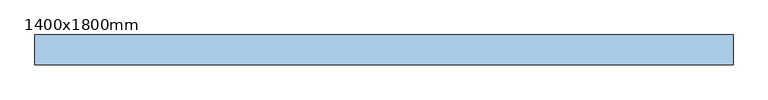
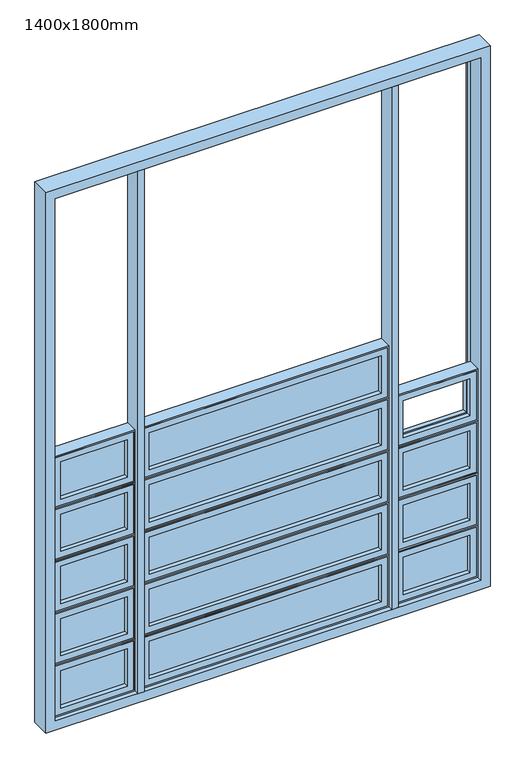
"""IFC4 building model written with IfcOpenShell, lengths in millimetres: window geometry, Janela Basculante 01 : 1400x1800mm."""

import ifcopenshell
import ifcopenshell.guid

model = None  # the IFC model being written
_history = None  # IfcOwnerHistory: only IFC2X3 demands one
_inside = {}  # id of a spatial element -> (the spatial element, [elements in it])
_under = {}  # id of a project, library or spatial element -> (it, [spatial elements below it])
_declared = {}  # id of a project -> (the project, [libraries it declares])
_typed = {}  # id of a type object -> (the type object, [elements of that type])
_made_of = {}  # id of a material, layer set ... -> (it, [elements and type objects made of it])


def new_model(schema):
    """Start an empty IFC model of exactly this schema.

    Asked for "IFC4X3", IfcOpenShell would pick the latest addendum, in which some entities
    have other attributes; the version numbers below select the first issue.
    IFC2X3 requires an IfcOwnerHistory on every rooted entity: one is made here for all.
    """
    global model, _history
    if schema == "IFC4X3":
        model = ifcopenshell.file(schema_version=(4, 3, 0, 0))
    else:
        model = ifcopenshell.file(schema=schema)
    _inside.clear()
    _under.clear()
    _declared.clear()
    _typed.clear()
    _made_of.clear()
    _history = None
    if model.schema == "IFC2X3":
        org = make("IfcOrganization", Name="unknown")
        user = make(
            "IfcPersonAndOrganization",
            ThePerson=make("IfcPerson", FamilyName="unknown"),
            TheOrganization=org,
        )
        app = make(
            "IfcApplication",
            ApplicationDeveloper=org,
            Version="unknown",
            ApplicationFullName="unknown",
            ApplicationIdentifier="unknown",
        )
        _history = make(
            "IfcOwnerHistory",
            OwningUser=user,
            OwningApplication=app,
            ChangeAction="ADDED",
            CreationDate=0,
        )
    return model


def make(cls, **values):
    """One entity of the class cls with the attributes given. An attribute that is None is left unset."""
    return model.create_entity(
        cls, **{name: value for name, value in values.items() if value is not None}
    )


def rooted(cls, **values):
    """An entity with a GlobalId (a new one), such as an element, a storey or a relation."""
    return make(cls, GlobalId=ifcopenshell.guid.new(), OwnerHistory=_history, **values)


def si_unit(unit_type, name, prefix=None):
    """IfcSIUnit, for example si_unit("LENGTHUNIT", "METRE", prefix="MILLI")."""
    return make("IfcSIUnit", UnitType=unit_type, Prefix=prefix, Name=name)


def assignment(units):
    """IfcUnitAssignment: the units of a project."""
    return None if units is None else make("IfcUnitAssignment", Units=units)


def point(xyz):
    """IfcCartesianPoint."""
    return None if xyz is None else make("IfcCartesianPoint", Coordinates=xyz)


def direction(xyz):
    """IfcDirection."""
    return None if xyz is None else make("IfcDirection", DirectionRatios=xyz)


def frame(location, z_axis=None, x_axis=None):
    """IfcAxis2Placement3D, a coordinate frame: its origin and axes. An axis left out is left unset."""
    return make(
        "IfcAxis2Placement3D",
        Location=point(location),
        Axis=direction(z_axis),
        RefDirection=direction(x_axis),
    )


def origin():
    """The frame at (0, 0, 0) with its axes left unset."""
    return frame((0.0, 0.0, 0.0))


def place(relative_to, where):
    """IfcLocalPlacement: puts the frame where relative to a parent placement (None: the world)."""
    return make(
        "IfcLocalPlacement", PlacementRelTo=relative_to, RelativePlacement=where
    )


def context(
    kind, dimensions, precision=None, world=None, true_north=None, identifier=None
):
    """IfcGeometricRepresentationContext, for example the 3D "Model" context."""
    return make(
        "IfcGeometricRepresentationContext",
        ContextIdentifier=identifier,
        ContextType=kind,
        CoordinateSpaceDimension=dimensions,
        Precision=precision,
        WorldCoordinateSystem=world,
        TrueNorth=true_north,
    )


def project(units=None, contexts=None):
    """IfcProject with its units and contexts."""
    return rooted(
        "IfcProject",
        Name="project",
        RepresentationContexts=contexts,
        UnitsInContext=assignment(units),
    )


def spatial(cls, under=None, at=None, **own):
    """A site, building, storey or space (cls), placed at a placement, below another one or the project."""
    s = rooted(cls, ObjectPlacement=at, **own)
    if under is not None:
        _under.setdefault(under.id(), (under, []))[1].append(s)
    return s


def polyline(points):
    """IfcPolyline through the points."""
    return make("IfcPolyline", Points=[point(p) for p in points])


def outline(outer, holes=None, kind="AREA"):
    """IfcArbitraryClosedProfileDef: a profile drawn as a closed curve; with holes, ...WithVoids."""
    if holes is None:
        return make("IfcArbitraryClosedProfileDef", ProfileType=kind, OuterCurve=outer)
    return make(
        "IfcArbitraryProfileDefWithVoids",
        ProfileType=kind,
        OuterCurve=outer,
        InnerCurves=holes,
    )


def extrude(swept, where, along, depth):
    """IfcExtrudedAreaSolid: the profile swept, set in the frame where, extruded along a direction by depth."""
    return make(
        "IfcExtrudedAreaSolid",
        SweptArea=swept,
        Position=where,
        ExtrudedDirection=direction(along),
        Depth=depth,
    )


def faces_of(points, faces, orient=None, outer=None):
    """IfcFace entities. A face is a list of loops; a loop is a list of indices into points, from 0.

    orient and outer hold one flag for each loop. By default every Orientation is true, the
    first loop of a face is its IfcFaceOuterBound and the others are IfcFaceBound.
    """
    made = []
    for i, loops in enumerate(faces):
        bounds = []
        for j, loop in enumerate(loops):
            is_outer = j == 0 if outer is None else outer[i][j]
            bounds.append(
                make(
                    "IfcFaceOuterBound" if is_outer else "IfcFaceBound",
                    Bound=make("IfcPolyLoop", Polygon=[points[k] for k in loop]),
                    Orientation=True if orient is None else orient[i][j],
                )
            )
        made.append(make("IfcFace", Bounds=bounds))
    return made


def faceted_brep(points, faces, orient=None, outer=None, voids=None):
    """IfcFacetedBrep: a solid bounded by flat faces; with voids (closed shells), ...WithVoids."""
    shared = [point(p) for p in points]
    hull = make("IfcClosedShell", CfsFaces=faces_of(shared, faces, orient, outer))
    if voids is None:
        return make("IfcFacetedBrep", Outer=hull)
    return make(
        "IfcFacetedBrepWithVoids",
        Outer=hull,
        Voids=[
            make(cls, CfsFaces=faces_of(shared, fs, o, b)) for cls, fs, o, b in voids
        ],
    )


def shape(context_of_items, identifier, shape_type, items):
    """IfcShapeRepresentation: the items that make up one representation, for example the "Body"."""
    return make(
        "IfcShapeRepresentation",
        ContextOfItems=context_of_items,
        RepresentationIdentifier=identifier,
        RepresentationType=shape_type,
        Items=items,
    )


def source(mapping_origin, context_of_items, identifier, shape_type, items):
    """IfcRepresentationMap: a shape defined once, which mapped items show again and again."""
    return make(
        "IfcRepresentationMap",
        MappingOrigin=mapping_origin,
        MappedRepresentation=shape(context_of_items, identifier, shape_type, items),
    )


def transform(
    local_origin,
    x_axis=None,
    y_axis=None,
    z_axis=None,
    scale=None,
    scale2=None,
    scale3=None,
    uniform=True,
):
    """IfcCartesianTransformationOperator3D, or its non-uniform kind. x_axis, y_axis, z_axis: its Axis1, 2, 3."""
    if uniform:
        return make(
            "IfcCartesianTransformationOperator3D",
            Axis1=direction(x_axis),
            Axis2=direction(y_axis),
            LocalOrigin=point(local_origin),
            Scale=scale,
            Axis3=direction(z_axis),
        )
    return make(
        "IfcCartesianTransformationOperator3DnonUniform",
        Axis1=direction(x_axis),
        Axis2=direction(y_axis),
        LocalOrigin=point(local_origin),
        Scale=scale,
        Axis3=direction(z_axis),
        Scale2=scale2,
        Scale3=scale3,
    )


def mapped(mapping_source, mapping_target):
    """IfcMappedItem: shows the shape of a source again, moved by a transform."""
    return make(
        "IfcMappedItem", MappingSource=mapping_source, MappingTarget=mapping_target
    )


def made_of(thing, what):
    """Note that an element or type object is made of a material, layer set ...; save() writes the relation."""
    if what is not None:
        _made_of.setdefault(what.id(), (what, []))[1].append(thing)
    return thing


def element(
    cls,
    number,
    at=None,
    inside=None,
    cuts=None,
    type_object=None,
    material=None,
    context=None,
    identifier="Body",
    shape_type=None,
    held_by="IfcProductDefinitionShape",
    body=None,
    shapes=None,
    **own,
):
    """One element of the class cls, such as IfcWall. Its Tag is "e" and its number.

    at: its placement. inside: the storey or other place that contains it. cuts: it is an
    opening in that element (IfcRelVoidsElement). A single representation is given by context,
    identifier, shape_type and body (its items); several are given by shapes. held_by: the class
    of the entity that holds the representations. save() writes the other relations.
    """
    e = rooted(cls, Tag="e%d" % number, ObjectPlacement=at, **own)
    if body is not None:
        shapes = [shape(context, identifier, shape_type, body)]
    if shapes is not None:
        e.Representation = make(held_by, Representations=shapes)
    if inside is not None:
        _inside.setdefault(inside.id(), (inside, []))[1].append(e)
    if cuts is not None:
        rooted(
            "IfcRelVoidsElement", RelatingBuildingElement=cuts, RelatedOpeningElement=e
        )
    if type_object is not None:
        _typed.setdefault(type_object.id(), (type_object, []))[1].append(e)
    return made_of(e, material)


def aggregate(whole, parts):
    """IfcRelAggregates: a whole, such as a stair, and the parts it consists of."""
    return rooted("IfcRelAggregates", RelatingObject=whole, RelatedObjects=parts)


def save(model, path):
    """Write the relations noted so far, then the file.

    IfcRelAggregates (storeys below a building ...), IfcRelContainedInSpatialStructure (elements
    in a storey), IfcRelDefinesByType, IfcRelAssociatesMaterial and IfcRelDeclares: one each for
    every whole, place, type object, material and project.
    """
    for whole, parts in _under.values():
        aggregate(whole, parts)
    for where, things in _inside.values():
        rooted(
            "IfcRelContainedInSpatialStructure",
            RelatedElements=things,
            RelatingStructure=where,
        )
    for kind, things in _typed.values():
        rooted("IfcRelDefinesByType", RelatedObjects=things, RelatingType=kind)
    for what, things in _made_of.values():
        rooted("IfcRelAssociatesMaterial", RelatedObjects=things, RelatingMaterial=what)
    for by, libraries in _declared.values():
        rooted("IfcRelDeclares", RelatingContext=by, RelatedDefinitions=libraries)
    model.write(path)


def window_1400x1800mm_1618d2dc(model_context):
    return source(origin(), model_context, "Body", "SolidModel", [
        faceted_brep([(435.0, -50.6, 1251.0), (435.0, -50.6, 1127.0), (435.0, -36.6, 1127.0), (435.0, -36.6, 1251.0), (428.0, -36.6, 1258.0), (428.0, -36.6, 1120.0), (428.0, -29.6, 1120.0), (428.0, -29.6, 1258.0), (435.0, -29.6, 1251.0), (435.0, -29.6, 1127.0), (435.0, -15.6, 1127.0), (435.0, -15.6, 1251.0), (415.0, -15.6, 1271.0), (415.0, -15.6, 1107.0), (415.0, -50.6, 1107.0), (415.0, -50.6, 1271.0), (645.0, -50.6, 1127.0), (645.0, -36.6, 1127.0), (652.0, -36.6, 1120.0), (652.0, -29.6, 1120.0), (645.0, -29.6, 1127.0), (645.0, -15.6, 1127.0), (665.0, -15.6, 1107.0), (665.0, -50.6, 1107.0), (645.0, -50.6, 1251.0), (645.0, -36.6, 1251.0), (652.0, -36.6, 1258.0), (652.0, -29.6, 1258.0), (645.0, -29.6, 1251.0), (645.0, -15.6, 1251.0), (665.0, -15.6, 1271.0), (665.0, -50.6, 1271.0)], [[[0, 1, 2, 3]], [[4, 5, 6, 7]], [[8, 9, 10, 11]], [[12, 13, 14, 15]], [[1, 16, 17, 2]], [[5, 18, 19, 6]], [[9, 20, 21, 10]], [[13, 22, 23, 14]], [[16, 24, 25, 17]], [[18, 26, 27, 19]], [[20, 28, 29, 21]], [[22, 30, 31, 23]], [[15, 14, 23, 31], [1, 0, 24, 16]], [[24, 0, 3, 25]], [[5, 4, 26, 18], [3, 2, 17, 25]], [[26, 4, 7, 27]], [[7, 6, 19, 27], [9, 8, 28, 20]], [[28, 8, 11, 29]], [[13, 12, 30, 22], [11, 10, 21, 29]], [[30, 12, 15, 31]]]),
        faceted_brep([(415.0, -50.6, 1271.0), (415.0, -50.6, 1107.0), (415.0, -15.6, 1107.0), (415.0, -15.6, 1271.0), (420.0, -15.6, 1266.0), (420.0, -15.6, 1112.0), (420.0, -10.6, 1112.0), (420.0, -10.6, 1266.0), (410.0, -10.6, 1276.0), (410.0, -10.6, 1102.0), (410.0, -50.6, 1102.0), (410.0, -50.6, 1276.0), (665.0, -50.6, 1107.0), (665.0, -15.6, 1107.0), (660.0, -15.6, 1112.0), (660.0, -10.6, 1112.0), (670.0, -10.6, 1102.0), (670.0, -50.6, 1102.0), (665.0, -50.6, 1271.0), (665.0, -15.6, 1271.0), (660.0, -15.6, 1266.0), (660.0, -10.6, 1266.0), (670.0, -10.6, 1276.0), (670.0, -50.6, 1276.0)], [[[0, 1, 2, 3]], [[4, 5, 6, 7]], [[8, 9, 10, 11]], [[1, 12, 13, 2]], [[5, 14, 15, 6]], [[9, 16, 17, 10]], [[12, 18, 19, 13]], [[14, 20, 21, 15]], [[16, 22, 23, 17]], [[11, 10, 17, 23], [1, 0, 18, 12]], [[18, 0, 3, 19]], [[3, 2, 13, 19], [5, 4, 20, 14]], [[20, 4, 7, 21]], [[9, 8, 22, 16], [7, 6, 15, 21]], [[22, 8, 11, 23]]]),
        extrude(outline(polyline([(652.0, -29.6), (652.0, -36.6), (428.0, -36.6), (428.0, -29.6), (652.0, -29.6)])), frame((0.0, 0.0, 946.0), z_axis=(0.0, 0.0, 1.0), x_axis=(1.0, 0.0, 0.0)), (0.0, 0.0, 1.0), 138.0),
        faceted_brep([(435.0, -50.6, 1077.0), (435.0, -50.6, 953.0), (435.0, -36.6, 953.0), (435.0, -36.6, 1077.0), (428.0, -36.6, 1084.0), (428.0, -36.6, 946.0), (428.0, -29.6, 946.0), (428.0, -29.6, 1084.0), (435.0, -29.6, 1077.0), (435.0, -29.6, 953.0), (435.0, -15.6, 953.0), (435.0, -15.6, 1077.0), (415.0, -15.6, 1097.0), (415.0, -15.6, 933.0), (415.0, -50.6, 933.0), (415.0, -50.6, 1097.0), (645.0, -50.6, 953.0), (645.0, -36.6, 953.0), (652.0, -36.6, 946.0), (652.0, -29.6, 946.0), (645.0, -29.6, 953.0), (645.0, -15.6, 953.0), (665.0, -15.6, 933.0), (665.0, -50.6, 933.0), (645.0, -50.6, 1077.0), (645.0, -36.6, 1077.0), (652.0, -36.6, 1084.0), (652.0, -29.6, 1084.0), (645.0, -29.6, 1077.0), (645.0, -15.6, 1077.0), (665.0, -15.6, 1097.0), (665.0, -50.6, 1097.0)], [[[0, 1, 2, 3]], [[4, 5, 6, 7]], [[8, 9, 10, 11]], [[12, 13, 14, 15]], [[1, 16, 17, 2]], [[5, 18, 19, 6]], [[9, 20, 21, 10]], [[13, 22, 23, 14]], [[16, 24, 25, 17]], [[18, 26, 27, 19]], [[20, 28, 29, 21]], [[22, 30, 31, 23]], [[15, 14, 23, 31], [1, 0, 24, 16]], [[24, 0, 3, 25]], [[5, 4, 26, 18], [3, 2, 17, 25]], [[26, 4, 7, 27]], [[7, 6, 19, 27], [9, 8, 28, 20]], [[28, 8, 11, 29]], [[13, 12, 30, 22], [11, 10, 21, 29]], [[30, 12, 15, 31]]]),
        faceted_brep([(415.0, -50.6, 1097.0), (415.0, -50.6, 933.0), (415.0, -15.6, 933.0), (415.0, -15.6, 1097.0), (420.0, -15.6, 1092.0), (420.0, -15.6, 938.0), (420.0, -10.6, 938.0), (420.0, -10.6, 1092.0), (410.0, -10.6, 1102.0), (410.0, -10.6, 928.0), (410.0, -50.6, 928.0), (410.0, -50.6, 1102.0), (665.0, -50.6, 933.0), (665.0, -15.6, 933.0), (660.0, -15.6, 938.0), (660.0, -10.6, 938.0), (670.0, -10.6, 928.0), (670.0, -50.6, 928.0), (665.0, -50.6, 1097.0), (665.0, -15.6, 1097.0), (660.0, -15.6, 1092.0), (660.0, -10.6, 1092.0), (670.0, -10.6, 1102.0), (670.0, -50.6, 1102.0)], [[[0, 1, 2, 3]], [[4, 5, 6, 7]], [[8, 9, 10, 11]], [[1, 12, 13, 2]], [[5, 14, 15, 6]], [[9, 16, 17, 10]], [[12, 18, 19, 13]], [[14, 20, 21, 15]], [[16, 22, 23, 17]], [[11, 10, 17, 23], [1, 0, 18, 12]], [[18, 0, 3, 19]], [[3, 2, 13, 19], [5, 4, 20, 14]], [[20, 4, 7, 21]], [[9, 8, 22, 16], [7, 6, 15, 21]], [[22, 8, 11, 23]]]),
        extrude(outline(polyline([(-372.0, -29.6), (372.0, -29.6), (372.0, -36.6), (-372.0, -36.6), (-372.0, -29.6)])), frame((0.0, 0.0, 1294.0), z_axis=(0.0, 0.0, 1.0), x_axis=(1.0, 0.0, 0.0)), (0.0, 0.0, 1.0), 138.0),
        faceted_brep([(365.0, -50.6, 1425.0), (365.0, -36.6, 1425.0), (365.0, -36.6, 1301.0), (365.0, -50.6, 1301.0), (372.0, -36.6, 1432.0), (372.0, -29.6, 1432.0), (372.0, -29.6, 1294.0), (372.0, -36.6, 1294.0), (365.0, -29.6, 1425.0), (365.0, -15.6, 1425.0), (365.0, -15.6, 1301.0), (365.0, -29.6, 1301.0), (385.0, -15.6, 1445.0), (385.0, -50.6, 1445.0), (385.0, -50.6, 1281.0), (385.0, -15.6, 1281.0), (-365.0, -36.6, 1301.0), (-365.0, -50.6, 1301.0), (-372.0, -29.6, 1294.0), (-372.0, -36.6, 1294.0), (-365.0, -15.6, 1301.0), (-365.0, -29.6, 1301.0), (-385.0, -50.6, 1281.0), (-385.0, -15.6, 1281.0), (-365.0, -36.6, 1425.0), (-365.0, -50.6, 1425.0), (-372.0, -29.6, 1432.0), (-372.0, -36.6, 1432.0), (-365.0, -15.6, 1425.0), (-365.0, -29.6, 1425.0), (-385.0, -50.6, 1445.0), (-385.0, -15.6, 1445.0)], [[[0, 1, 2, 3]], [[4, 5, 6, 7]], [[8, 9, 10, 11]], [[12, 13, 14, 15]], [[3, 2, 16, 17]], [[7, 6, 18, 19]], [[11, 10, 20, 21]], [[15, 14, 22, 23]], [[17, 16, 24, 25]], [[19, 18, 26, 27]], [[21, 20, 28, 29]], [[23, 22, 30, 31]], [[13, 30, 22, 14], [3, 17, 25, 0]], [[25, 24, 1, 0]], [[7, 19, 27, 4], [1, 24, 16, 2]], [[27, 26, 5, 4]], [[5, 26, 18, 6], [11, 21, 29, 8]], [[29, 28, 9, 8]], [[15, 23, 31, 12], [9, 28, 20, 10]], [[31, 30, 13, 12]]]),
        faceted_brep([(385.0, -50.6, 1445.0), (385.0, -15.6, 1445.0), (385.0, -15.6, 1281.0), (385.0, -50.6, 1281.0), (380.0, -15.6, 1440.0), (380.0, -10.6, 1440.0), (380.0, -10.6, 1286.0), (380.0, -15.6, 1286.0), (390.0, -10.6, 1450.0), (390.0, -50.6, 1450.0), (390.0, -50.6, 1276.0), (390.0, -10.6, 1276.0), (-385.0, -15.6, 1281.0), (-385.0, -50.6, 1281.0), (-380.0, -10.6, 1286.0), (-380.0, -15.6, 1286.0), (-390.0, -50.6, 1276.0), (-390.0, -10.6, 1276.0), (-385.0, -15.6, 1445.0), (-385.0, -50.6, 1445.0), (-380.0, -10.6, 1440.0), (-380.0, -15.6, 1440.0), (-390.0, -50.6, 1450.0), (-390.0, -10.6, 1450.0)], [[[0, 1, 2, 3]], [[4, 5, 6, 7]], [[8, 9, 10, 11]], [[3, 2, 12, 13]], [[7, 6, 14, 15]], [[11, 10, 16, 17]], [[13, 12, 18, 19]], [[15, 14, 20, 21]], [[17, 16, 22, 23]], [[9, 22, 16, 10], [3, 13, 19, 0]], [[19, 18, 1, 0]], [[1, 18, 12, 2], [7, 15, 21, 4]], [[21, 20, 5, 4]], [[11, 17, 23, 8], [5, 20, 14, 6]], [[23, 22, 9, 8]]]),
        extrude(outline(polyline([(-372.0, -29.6), (372.0, -29.6), (372.0, -36.6), (-372.0, -36.6), (-372.0, -29.6)])), frame((0.0, 0.0, 1120.0), z_axis=(0.0, 0.0, 1.0), x_axis=(1.0, 0.0, 0.0)), (0.0, 0.0, 1.0), 138.0),
        faceted_brep([(365.0, -50.6, 1251.0), (365.0, -36.6, 1251.0), (365.0, -36.6, 1127.0), (365.0, -50.6, 1127.0), (372.0, -36.6, 1258.0), (372.0, -29.6, 1258.0), (372.0, -29.6, 1120.0), (372.0, -36.6, 1120.0), (365.0, -29.6, 1251.0), (365.0, -15.6, 1251.0), (365.0, -15.6, 1127.0), (365.0, -29.6, 1127.0), (385.0, -15.6, 1271.0), (385.0, -50.6, 1271.0), (385.0, -50.6, 1107.0), (385.0, -15.6, 1107.0), (-365.0, -36.6, 1127.0), (-365.0, -50.6, 1127.0), (-372.0, -29.6, 1120.0), (-372.0, -36.6, 1120.0), (-365.0, -15.6, 1127.0), (-365.0, -29.6, 1127.0), (-385.0, -50.6, 1107.0), (-385.0, -15.6, 1107.0), (-365.0, -36.6, 1251.0), (-365.0, -50.6, 1251.0), (-372.0, -29.6, 1258.0), (-372.0, -36.6, 1258.0), (-365.0, -15.6, 1251.0), (-365.0, -29.6, 1251.0), (-385.0, -50.6, 1271.0), (-385.0, -15.6, 1271.0)], [[[0, 1, 2, 3]], [[4, 5, 6, 7]], [[8, 9, 10, 11]], [[12, 13, 14, 15]], [[3, 2, 16, 17]], [[7, 6, 18, 19]], [[11, 10, 20, 21]], [[15, 14, 22, 23]], [[17, 16, 24, 25]], [[19, 18, 26, 27]], [[21, 20, 28, 29]], [[23, 22, 30, 31]], [[13, 30, 22, 14], [3, 17, 25, 0]], [[25, 24, 1, 0]], [[7, 19, 27, 4], [1, 24, 16, 2]], [[27, 26, 5, 4]], [[5, 26, 18, 6], [11, 21, 29, 8]], [[29, 28, 9, 8]], [[15, 23, 31, 12], [9, 28, 20, 10]], [[31, 30, 13, 12]]]),
        faceted_brep([(385.0, -50.6, 1271.0), (385.0, -15.6, 1271.0), (385.0, -15.6, 1107.0), (385.0, -50.6, 1107.0), (380.0, -15.6, 1266.0), (380.0, -10.6, 1266.0), (380.0, -10.6, 1112.0), (380.0, -15.6, 1112.0), (390.0, -10.6, 1276.0), (390.0, -50.6, 1276.0), (390.0, -50.6, 1102.0), (390.0, -10.6, 1102.0), (-385.0, -15.6, 1107.0), (-385.0, -50.6, 1107.0), (-380.0, -10.6, 1112.0), (-380.0, -15.6, 1112.0), (-390.0, -50.6, 1102.0), (-390.0, -10.6, 1102.0), (-385.0, -15.6, 1271.0), (-385.0, -50.6, 1271.0), (-380.0, -10.6, 1266.0), (-380.0, -15.6, 1266.0), (-390.0, -50.6, 1276.0), (-390.0, -10.6, 1276.0)], [[[0, 1, 2, 3]], [[4, 5, 6, 7]], [[8, 9, 10, 11]], [[3, 2, 12, 13]], [[7, 6, 14, 15]], [[11, 10, 16, 17]], [[13, 12, 18, 19]], [[15, 14, 20, 21]], [[17, 16, 22, 23]], [[9, 22, 16, 10], [3, 13, 19, 0]], [[19, 18, 1, 0]], [[1, 18, 12, 2], [7, 15, 21, 4]], [[21, 20, 5, 4]], [[11, 17, 23, 8], [5, 20, 14, 6]], [[23, 22, 9, 8]]]),
        extrude(outline(polyline([(-372.0, -29.6), (372.0, -29.6), (372.0, -36.6), (-372.0, -36.6), (-372.0, -29.6)])), frame((0.0, 0.0, 946.0), z_axis=(0.0, 0.0, 1.0), x_axis=(1.0, 0.0, 0.0)), (0.0, 0.0, 1.0), 138.0),
        faceted_brep([(365.0, -50.6, 1077.0), (365.0, -36.6, 1077.0), (365.0, -36.6, 953.0), (365.0, -50.6, 953.0), (372.0, -36.6, 1084.0), (372.0, -29.6, 1084.0), (372.0, -29.6, 946.0), (372.0, -36.6, 946.0), (365.0, -29.6, 1077.0), (365.0, -15.6, 1077.0), (365.0, -15.6, 953.0), (365.0, -29.6, 953.0), (385.0, -15.6, 1097.0), (385.0, -50.6, 1097.0), (385.0, -50.6, 933.0), (385.0, -15.6, 933.0), (-365.0, -36.6, 953.0), (-365.0, -50.6, 953.0), (-372.0, -29.6, 946.0), (-372.0, -36.6, 946.0), (-365.0, -15.6, 953.0), (-365.0, -29.6, 953.0), (-385.0, -50.6, 933.0), (-385.0, -15.6, 933.0), (-365.0, -36.6, 1077.0), (-365.0, -50.6, 1077.0), (-372.0, -29.6, 1084.0), (-372.0, -36.6, 1084.0), (-365.0, -15.6, 1077.0), (-365.0, -29.6, 1077.0), (-385.0, -50.6, 1097.0), (-385.0, -15.6, 1097.0)], [[[0, 1, 2, 3]], [[4, 5, 6, 7]], [[8, 9, 10, 11]], [[12, 13, 14, 15]], [[3, 2, 16, 17]], [[7, 6, 18, 19]], [[11, 10, 20, 21]], [[15, 14, 22, 23]], [[17, 16, 24, 25]], [[19, 18, 26, 27]], [[21, 20, 28, 29]], [[23, 22, 30, 31]], [[13, 30, 22, 14], [3, 17, 25, 0]], [[25, 24, 1, 0]], [[7, 19, 27, 4], [1, 24, 16, 2]], [[27, 26, 5, 4]], [[5, 26, 18, 6], [11, 21, 29, 8]], [[29, 28, 9, 8]], [[15, 23, 31, 12], [9, 28, 20, 10]], [[31, 30, 13, 12]]]),
        faceted_brep([(385.0, -50.6, 1097.0), (385.0, -15.6, 1097.0), (385.0, -15.6, 933.0), (385.0, -50.6, 933.0), (380.0, -15.6, 1092.0), (380.0, -10.6, 1092.0), (380.0, -10.6, 938.0), (380.0, -15.6, 938.0), (390.0, -10.6, 1102.0), (390.0, -50.6, 1102.0), (390.0, -50.6, 928.0), (390.0, -10.6, 928.0), (-385.0, -15.6, 933.0), (-385.0, -50.6, 933.0), (-380.0, -10.6, 938.0), (-380.0, -15.6, 938.0), (-390.0, -50.6, 928.0), (-390.0, -10.6, 928.0), (-385.0, -15.6, 1097.0), (-385.0, -50.6, 1097.0), (-380.0, -10.6, 1092.0), (-380.0, -15.6, 1092.0), (-390.0, -50.6, 1102.0), (-390.0, -10.6, 1102.0)], [[[0, 1, 2, 3]], [[4, 5, 6, 7]], [[8, 9, 10, 11]], [[3, 2, 12, 13]], [[7, 6, 14, 15]], [[11, 10, 16, 17]], [[13, 12, 18, 19]], [[15, 14, 20, 21]], [[17, 16, 22, 23]], [[9, 22, 16, 10], [3, 13, 19, 0]], [[19, 18, 1, 0]], [[1, 18, 12, 2], [7, 15, 21, 4]], [[21, 20, 5, 4]], [[11, 17, 23, 8], [5, 20, 14, 6]], [[23, 22, 9, 8]]]),
        extrude(outline(polyline([(-428.0, -29.6), (-428.0, -36.6), (-652.0, -36.6), (-652.0, -29.6), (-428.0, -29.6)])), frame((0.0, 0.0, 1294.0), z_axis=(0.0, 0.0, 1.0), x_axis=(1.0, 0.0, 0.0)), (0.0, 0.0, 1.0), 138.0),
        faceted_brep([(-645.0, -50.6, 1425.0), (-645.0, -50.6, 1301.0), (-645.0, -36.6, 1301.0), (-645.0, -36.6, 1425.0), (-652.0, -36.6, 1432.0), (-652.0, -36.6, 1294.0), (-652.0, -29.6, 1294.0), (-652.0, -29.6, 1432.0), (-645.0, -29.6, 1425.0), (-645.0, -29.6, 1301.0), (-645.0, -15.6, 1301.0), (-645.0, -15.6, 1425.0), (-665.0, -15.6, 1445.0), (-665.0, -15.6, 1281.0), (-665.0, -50.6, 1281.0), (-665.0, -50.6, 1445.0), (-435.0, -50.6, 1301.0), (-435.0, -36.6, 1301.0), (-428.0, -36.6, 1294.0), (-428.0, -29.6, 1294.0), (-435.0, -29.6, 1301.0), (-435.0, -15.6, 1301.0), (-415.0, -15.6, 1281.0), (-415.0, -50.6, 1281.0), (-435.0, -50.6, 1425.0), (-435.0, -36.6, 1425.0), (-428.0, -36.6, 1432.0), (-428.0, -29.6, 1432.0), (-435.0, -29.6, 1425.0), (-435.0, -15.6, 1425.0), (-415.0, -15.6, 1445.0), (-415.0, -50.6, 1445.0)], [[[0, 1, 2, 3]], [[4, 5, 6, 7]], [[8, 9, 10, 11]], [[12, 13, 14, 15]], [[1, 16, 17, 2]], [[5, 18, 19, 6]], [[9, 20, 21, 10]], [[13, 22, 23, 14]], [[16, 24, 25, 17]], [[18, 26, 27, 19]], [[20, 28, 29, 21]], [[22, 30, 31, 23]], [[15, 14, 23, 31], [1, 0, 24, 16]], [[24, 0, 3, 25]], [[5, 4, 26, 18], [3, 2, 17, 25]], [[26, 4, 7, 27]], [[7, 6, 19, 27], [9, 8, 28, 20]], [[28, 8, 11, 29]], [[13, 12, 30, 22], [11, 10, 21, 29]], [[30, 12, 15, 31]]]),
        faceted_brep([(-665.0, -50.6, 1445.0), (-665.0, -50.6, 1281.0), (-665.0, -15.6, 1281.0), (-665.0, -15.6, 1445.0), (-660.0, -15.6, 1440.0), (-660.0, -15.6, 1286.0), (-660.0, -10.6, 1286.0), (-660.0, -10.6, 1440.0), (-670.0, -10.6, 1450.0), (-670.0, -10.6, 1276.0), (-670.0, -50.6, 1276.0), (-670.0, -50.6, 1450.0), (-415.0, -50.6, 1281.0), (-415.0, -15.6, 1281.0), (-420.0, -15.6, 1286.0), (-420.0, -10.6, 1286.0), (-410.0, -10.6, 1276.0), (-410.0, -50.6, 1276.0), (-415.0, -50.6, 1445.0), (-415.0, -15.6, 1445.0), (-420.0, -15.6, 1440.0), (-420.0, -10.6, 1440.0), (-410.0, -10.6, 1450.0), (-410.0, -50.6, 1450.0)], [[[0, 1, 2, 3]], [[4, 5, 6, 7]], [[8, 9, 10, 11]], [[1, 12, 13, 2]], [[5, 14, 15, 6]], [[9, 16, 17, 10]], [[12, 18, 19, 13]], [[14, 20, 21, 15]], [[16, 22, 23, 17]], [[11, 10, 17, 23], [1, 0, 18, 12]], [[18, 0, 3, 19]], [[3, 2, 13, 19], [5, 4, 20, 14]], [[20, 4, 7, 21]], [[9, 8, 22, 16], [7, 6, 15, 21]], [[22, 8, 11, 23]]]),
        extrude(outline(polyline([(-428.0, -29.6), (-428.0, -36.6), (-652.0, -36.6), (-652.0, -29.6), (-428.0, -29.6)])), frame((0.0, 0.0, 1120.0), z_axis=(0.0, 0.0, 1.0), x_axis=(1.0, 0.0, 0.0)), (0.0, 0.0, 1.0), 138.0),
        faceted_brep([(-645.0, -50.6, 1251.0), (-645.0, -50.6, 1127.0), (-645.0, -36.6, 1127.0), (-645.0, -36.6, 1251.0), (-652.0, -36.6, 1258.0), (-652.0, -36.6, 1120.0), (-652.0, -29.6, 1120.0), (-652.0, -29.6, 1258.0), (-645.0, -29.6, 1251.0), (-645.0, -29.6, 1127.0), (-645.0, -15.6, 1127.0), (-645.0, -15.6, 1251.0), (-665.0, -15.6, 1271.0), (-665.0, -15.6, 1107.0), (-665.0, -50.6, 1107.0), (-665.0, -50.6, 1271.0), (-435.0, -50.6, 1127.0), (-435.0, -36.6, 1127.0), (-428.0, -36.6, 1120.0), (-428.0, -29.6, 1120.0), (-435.0, -29.6, 1127.0), (-435.0, -15.6, 1127.0), (-415.0, -15.6, 1107.0), (-415.0, -50.6, 1107.0), (-435.0, -50.6, 1251.0), (-435.0, -36.6, 1251.0), (-428.0, -36.6, 1258.0), (-428.0, -29.6, 1258.0), (-435.0, -29.6, 1251.0), (-435.0, -15.6, 1251.0), (-415.0, -15.6, 1271.0), (-415.0, -50.6, 1271.0)], [[[0, 1, 2, 3]], [[4, 5, 6, 7]], [[8, 9, 10, 11]], [[12, 13, 14, 15]], [[1, 16, 17, 2]], [[5, 18, 19, 6]], [[9, 20, 21, 10]], [[13, 22, 23, 14]], [[16, 24, 25, 17]], [[18, 26, 27, 19]], [[20, 28, 29, 21]], [[22, 30, 31, 23]], [[15, 14, 23, 31], [1, 0, 24, 16]], [[24, 0, 3, 25]], [[5, 4, 26, 18], [3, 2, 17, 25]], [[26, 4, 7, 27]], [[7, 6, 19, 27], [9, 8, 28, 20]], [[28, 8, 11, 29]], [[13, 12, 30, 22], [11, 10, 21, 29]], [[30, 12, 15, 31]]]),
        faceted_brep([(-665.0, -50.6, 1271.0), (-665.0, -50.6, 1107.0), (-665.0, -15.6, 1107.0), (-665.0, -15.6, 1271.0), (-660.0, -15.6, 1266.0), (-660.0, -15.6, 1112.0), (-660.0, -10.6, 1112.0), (-660.0, -10.6, 1266.0), (-670.0, -10.6, 1276.0), (-670.0, -10.6, 1102.0), (-670.0, -50.6, 1102.0), (-670.0, -50.6, 1276.0), (-415.0, -50.6, 1107.0), (-415.0, -15.6, 1107.0), (-420.0, -15.6, 1112.0), (-420.0, -10.6, 1112.0), (-410.0, -10.6, 1102.0), (-410.0, -50.6, 1102.0), (-415.0, -50.6, 1271.0), (-415.0, -15.6, 1271.0), (-420.0, -15.6, 1266.0), (-420.0, -10.6, 1266.0), (-410.0, -10.6, 1276.0), (-410.0, -50.6, 1276.0)], [[[0, 1, 2, 3]], [[4, 5, 6, 7]], [[8, 9, 10, 11]], [[1, 12, 13, 2]], [[5, 14, 15, 6]], [[9, 16, 17, 10]], [[12, 18, 19, 13]], [[14, 20, 21, 15]], [[16, 22, 23, 17]], [[11, 10, 17, 23], [1, 0, 18, 12]], [[18, 0, 3, 19]], [[3, 2, 13, 19], [5, 4, 20, 14]], [[20, 4, 7, 21]], [[9, 8, 22, 16], [7, 6, 15, 21]], [[22, 8, 11, 23]]]),
        extrude(outline(polyline([(-428.0, -29.6), (-428.0, -36.6), (-652.0, -36.6), (-652.0, -29.6), (-428.0, -29.6)])), frame((0.0, 0.0, 946.0), z_axis=(0.0, 0.0, 1.0), x_axis=(1.0, 0.0, 0.0)), (0.0, 0.0, 1.0), 138.0),
        faceted_brep([(-645.0, -50.6, 1077.0), (-645.0, -50.6, 953.0), (-645.0, -36.6, 953.0), (-645.0, -36.6, 1077.0), (-652.0, -36.6, 1084.0), (-652.0, -36.6, 946.0), (-652.0, -29.6, 946.0), (-652.0, -29.6, 1084.0), (-645.0, -29.6, 1077.0), (-645.0, -29.6, 953.0), (-645.0, -15.6, 953.0), (-645.0, -15.6, 1077.0), (-665.0, -15.6, 1097.0), (-665.0, -15.6, 933.0), (-665.0, -50.6, 933.0), (-665.0, -50.6, 1097.0), (-435.0, -50.6, 953.0), (-435.0, -36.6, 953.0), (-428.0, -36.6, 946.0), (-428.0, -29.6, 946.0), (-435.0, -29.6, 953.0), (-435.0, -15.6, 953.0), (-415.0, -15.6, 933.0), (-415.0, -50.6, 933.0), (-435.0, -50.6, 1077.0), (-435.0, -36.6, 1077.0), (-428.0, -36.6, 1084.0), (-428.0, -29.6, 1084.0), (-435.0, -29.6, 1077.0), (-435.0, -15.6, 1077.0), (-415.0, -15.6, 1097.0), (-415.0, -50.6, 1097.0)], [[[0, 1, 2, 3]], [[4, 5, 6, 7]], [[8, 9, 10, 11]], [[12, 13, 14, 15]], [[1, 16, 17, 2]], [[5, 18, 19, 6]], [[9, 20, 21, 10]], [[13, 22, 23, 14]], [[16, 24, 25, 17]], [[18, 26, 27, 19]], [[20, 28, 29, 21]], [[22, 30, 31, 23]], [[15, 14, 23, 31], [1, 0, 24, 16]], [[24, 0, 3, 25]], [[5, 4, 26, 18], [3, 2, 17, 25]], [[26, 4, 7, 27]], [[7, 6, 19, 27], [9, 8, 28, 20]], [[28, 8, 11, 29]], [[13, 12, 30, 22], [11, 10, 21, 29]], [[30, 12, 15, 31]]]),
        faceted_brep([(-665.0, -50.6, 1097.0), (-665.0, -50.6, 933.0), (-665.0, -15.6, 933.0), (-665.0, -15.6, 1097.0), (-660.0, -15.6, 1092.0), (-660.0, -15.6, 938.0), (-660.0, -10.6, 938.0), (-660.0, -10.6, 1092.0), (-670.0, -10.6, 1102.0), (-670.0, -10.6, 928.0), (-670.0, -50.6, 928.0), (-670.0, -50.6, 1102.0), (-415.0, -50.6, 933.0), (-415.0, -15.6, 933.0), (-420.0, -15.6, 938.0), (-420.0, -10.6, 938.0), (-410.0, -10.6, 928.0), (-410.0, -50.6, 928.0), (-415.0, -50.6, 1097.0), (-415.0, -15.6, 1097.0), (-420.0, -15.6, 1092.0), (-420.0, -10.6, 1092.0), (-410.0, -10.6, 1102.0), (-410.0, -50.6, 1102.0)], [[[0, 1, 2, 3]], [[4, 5, 6, 7]], [[8, 9, 10, 11]], [[1, 12, 13, 2]], [[5, 14, 15, 6]], [[9, 16, 17, 10]], [[12, 18, 19, 13]], [[14, 20, 21, 15]], [[16, 22, 23, 17]], [[11, 10, 17, 23], [1, 0, 18, 12]], [[18, 0, 3, 19]], [[3, 2, 13, 19], [5, 4, 20, 14]], [[20, 4, 7, 21]], [[9, 8, 22, 16], [7, 6, 15, 21]], [[22, 8, 11, 23]]]),
        extrude(outline(polyline([(652.0, -29.6), (652.0, -36.6), (428.0, -36.6), (428.0, -29.6), (652.0, -29.6)])), frame((0.0, 0.0, 772.0), z_axis=(0.0, 0.0, 1.0), x_axis=(1.0, 0.0, 0.0)), (0.0, 0.0, 1.0), 138.0),
        faceted_brep([(435.0, -50.6, 903.0), (435.0, -50.6, 779.0), (435.0, -36.6, 779.0), (435.0, -36.6, 903.0), (428.0, -36.6, 910.0), (428.0, -36.6, 772.0), (428.0, -29.6, 772.0), (428.0, -29.6, 910.0), (435.0, -29.6, 903.0), (435.0, -29.6, 779.0), (435.0, -15.6, 779.0), (435.0, -15.6, 903.0), (415.0, -15.6, 923.0), (415.0, -15.6, 759.0), (415.0, -50.6, 759.0), (415.0, -50.6, 923.0), (645.0, -50.6, 779.0), (645.0, -36.6, 779.0), (652.0, -36.6, 772.0), (652.0, -29.6, 772.0), (645.0, -29.6, 779.0), (645.0, -15.6, 779.0), (665.0, -15.6, 759.0), (665.0, -50.6, 759.0), (645.0, -50.6, 903.0), (645.0, -36.6, 903.0), (652.0, -36.6, 910.0), (652.0, -29.6, 910.0), (645.0, -29.6, 903.0), (645.0, -15.6, 903.0), (665.0, -15.6, 923.0), (665.0, -50.6, 923.0)], [[[0, 1, 2, 3]], [[4, 5, 6, 7]], [[8, 9, 10, 11]], [[12, 13, 14, 15]], [[1, 16, 17, 2]], [[5, 18, 19, 6]], [[9, 20, 21, 10]], [[13, 22, 23, 14]], [[16, 24, 25, 17]], [[18, 26, 27, 19]], [[20, 28, 29, 21]], [[22, 30, 31, 23]], [[15, 14, 23, 31], [1, 0, 24, 16]], [[24, 0, 3, 25]], [[5, 4, 26, 18], [3, 2, 17, 25]], [[26, 4, 7, 27]], [[7, 6, 19, 27], [9, 8, 28, 20]], [[28, 8, 11, 29]], [[13, 12, 30, 22], [11, 10, 21, 29]], [[30, 12, 15, 31]]]),
        faceted_brep([(415.0, -50.6, 923.0), (415.0, -50.6, 759.0), (415.0, -15.6, 759.0), (415.0, -15.6, 923.0), (420.0, -15.6, 918.0), (420.0, -15.6, 764.0), (420.0, -10.6, 764.0), (420.0, -10.6, 918.0), (410.0, -10.6, 928.0), (410.0, -10.6, 754.0), (410.0, -50.6, 754.0), (410.0, -50.6, 928.0), (665.0, -50.6, 759.0), (665.0, -15.6, 759.0), (660.0, -15.6, 764.0), (660.0, -10.6, 764.0), (670.0, -10.6, 754.0), (670.0, -50.6, 754.0), (665.0, -50.6, 923.0), (665.0, -15.6, 923.0), (660.0, -15.6, 918.0), (660.0, -10.6, 918.0), (670.0, -10.6, 928.0), (670.0, -50.6, 928.0)], [[[0, 1, 2, 3]], [[4, 5, 6, 7]], [[8, 9, 10, 11]], [[1, 12, 13, 2]], [[5, 14, 15, 6]], [[9, 16, 17, 10]], [[12, 18, 19, 13]], [[14, 20, 21, 15]], [[16, 22, 23, 17]], [[11, 10, 17, 23], [1, 0, 18, 12]], [[18, 0, 3, 19]], [[3, 2, 13, 19], [5, 4, 20, 14]], [[20, 4, 7, 21]], [[9, 8, 22, 16], [7, 6, 15, 21]], [[22, 8, 11, 23]]]),
        extrude(outline(polyline([(652.0, -29.6), (652.0, -36.6), (428.0, -36.6), (428.0, -29.6), (652.0, -29.6)])), frame((0.0, 0.0, 598.0), z_axis=(0.0, 0.0, 1.0), x_axis=(1.0, 0.0, 0.0)), (0.0, 0.0, 1.0), 138.0),
        faceted_brep([(435.0, -50.6, 729.0), (435.0, -50.6, 605.0), (435.0, -36.6, 605.0), (435.0, -36.6, 729.0), (428.0, -36.6, 736.0), (428.0, -36.6, 598.0), (428.0, -29.6, 598.0), (428.0, -29.6, 736.0), (435.0, -29.6, 729.0), (435.0, -29.6, 605.0), (435.0, -15.6, 605.0), (435.0, -15.6, 729.0), (415.0, -15.6, 749.0), (415.0, -15.6, 585.0), (415.0, -50.6, 585.0), (415.0, -50.6, 749.0), (645.0, -50.6, 605.0), (645.0, -36.6, 605.0), (652.0, -36.6, 598.0), (652.0, -29.6, 598.0), (645.0, -29.6, 605.0), (645.0, -15.6, 605.0), (665.0, -15.6, 585.0), (665.0, -50.6, 585.0), (645.0, -50.6, 729.0), (645.0, -36.6, 729.0), (652.0, -36.6, 736.0), (652.0, -29.6, 736.0), (645.0, -29.6, 729.0), (645.0, -15.6, 729.0), (665.0, -15.6, 749.0), (665.0, -50.6, 749.0)], [[[0, 1, 2, 3]], [[4, 5, 6, 7]], [[8, 9, 10, 11]], [[12, 13, 14, 15]], [[1, 16, 17, 2]], [[5, 18, 19, 6]], [[9, 20, 21, 10]], [[13, 22, 23, 14]], [[16, 24, 25, 17]], [[18, 26, 27, 19]], [[20, 28, 29, 21]], [[22, 30, 31, 23]], [[15, 14, 23, 31], [1, 0, 24, 16]], [[24, 0, 3, 25]], [[5, 4, 26, 18], [3, 2, 17, 25]], [[26, 4, 7, 27]], [[7, 6, 19, 27], [9, 8, 28, 20]], [[28, 8, 11, 29]], [[13, 12, 30, 22], [11, 10, 21, 29]], [[30, 12, 15, 31]]]),
        faceted_brep([(415.0, -50.6, 749.0), (415.0, -50.6, 585.0), (415.0, -15.6, 585.0), (415.0, -15.6, 749.0), (420.0, -15.6, 744.0), (420.0, -15.6, 590.0), (420.0, -10.6, 590.0), (420.0, -10.6, 744.0), (410.0, -10.6, 754.0), (410.0, -10.6, 580.0), (410.0, -50.6, 580.0), (410.0, -50.6, 754.0), (665.0, -50.6, 585.0), (665.0, -15.6, 585.0), (660.0, -15.6, 590.0), (660.0, -10.6, 590.0), (670.0, -10.6, 580.0), (670.0, -50.6, 580.0), (665.0, -50.6, 749.0), (665.0, -15.6, 749.0), (660.0, -15.6, 744.0), (660.0, -10.6, 744.0), (670.0, -10.6, 754.0), (670.0, -50.6, 754.0)], [[[0, 1, 2, 3]], [[4, 5, 6, 7]], [[8, 9, 10, 11]], [[1, 12, 13, 2]], [[5, 14, 15, 6]], [[9, 16, 17, 10]], [[12, 18, 19, 13]], [[14, 20, 21, 15]], [[16, 22, 23, 17]], [[11, 10, 17, 23], [1, 0, 18, 12]], [[18, 0, 3, 19]], [[3, 2, 13, 19], [5, 4, 20, 14]], [[20, 4, 7, 21]], [[9, 8, 22, 16], [7, 6, 15, 21]], [[22, 8, 11, 23]]]),
        extrude(outline(polyline([(-372.0, -29.6), (372.0, -29.6), (372.0, -36.6), (-372.0, -36.6), (-372.0, -29.6)])), frame((0.0, 0.0, 772.0), z_axis=(0.0, 0.0, 1.0), x_axis=(1.0, 0.0, 0.0)), (0.0, 0.0, 1.0), 138.0),
        faceted_brep([(365.0, -50.6, 903.0), (365.0, -36.6, 903.0), (365.0, -36.6, 779.0), (365.0, -50.6, 779.0), (372.0, -36.6, 910.0), (372.0, -29.6, 910.0), (372.0, -29.6, 772.0), (372.0, -36.6, 772.0), (365.0, -29.6, 903.0), (365.0, -15.6, 903.0), (365.0, -15.6, 779.0), (365.0, -29.6, 779.0), (385.0, -15.6, 923.0), (385.0, -50.6, 923.0), (385.0, -50.6, 759.0), (385.0, -15.6, 759.0), (-365.0, -36.6, 779.0), (-365.0, -50.6, 779.0), (-372.0, -29.6, 772.0), (-372.0, -36.6, 772.0), (-365.0, -15.6, 779.0), (-365.0, -29.6, 779.0), (-385.0, -50.6, 759.0), (-385.0, -15.6, 759.0), (-365.0, -36.6, 903.0), (-365.0, -50.6, 903.0), (-372.0, -29.6, 910.0), (-372.0, -36.6, 910.0), (-365.0, -15.6, 903.0), (-365.0, -29.6, 903.0), (-385.0, -50.6, 923.0), (-385.0, -15.6, 923.0)], [[[0, 1, 2, 3]], [[4, 5, 6, 7]], [[8, 9, 10, 11]], [[12, 13, 14, 15]], [[3, 2, 16, 17]], [[7, 6, 18, 19]], [[11, 10, 20, 21]], [[15, 14, 22, 23]], [[17, 16, 24, 25]], [[19, 18, 26, 27]], [[21, 20, 28, 29]], [[23, 22, 30, 31]], [[13, 30, 22, 14], [3, 17, 25, 0]], [[25, 24, 1, 0]], [[7, 19, 27, 4], [1, 24, 16, 2]], [[27, 26, 5, 4]], [[5, 26, 18, 6], [11, 21, 29, 8]], [[29, 28, 9, 8]], [[15, 23, 31, 12], [9, 28, 20, 10]], [[31, 30, 13, 12]]]),
        faceted_brep([(385.0, -50.6, 923.0), (385.0, -15.6, 923.0), (385.0, -15.6, 759.0), (385.0, -50.6, 759.0), (380.0, -15.6, 918.0), (380.0, -10.6, 918.0), (380.0, -10.6, 764.0), (380.0, -15.6, 764.0), (390.0, -10.6, 928.0), (390.0, -50.6, 928.0), (390.0, -50.6, 754.0), (390.0, -10.6, 754.0), (-385.0, -15.6, 759.0), (-385.0, -50.6, 759.0), (-380.0, -10.6, 764.0), (-380.0, -15.6, 764.0), (-390.0, -50.6, 754.0), (-390.0, -10.6, 754.0), (-385.0, -15.6, 923.0), (-385.0, -50.6, 923.0), (-380.0, -10.6, 918.0), (-380.0, -15.6, 918.0), (-390.0, -50.6, 928.0), (-390.0, -10.6, 928.0)], [[[0, 1, 2, 3]], [[4, 5, 6, 7]], [[8, 9, 10, 11]], [[3, 2, 12, 13]], [[7, 6, 14, 15]], [[11, 10, 16, 17]], [[13, 12, 18, 19]], [[15, 14, 20, 21]], [[17, 16, 22, 23]], [[9, 22, 16, 10], [3, 13, 19, 0]], [[19, 18, 1, 0]], [[1, 18, 12, 2], [7, 15, 21, 4]], [[21, 20, 5, 4]], [[11, 17, 23, 8], [5, 20, 14, 6]], [[23, 22, 9, 8]]]),
        extrude(outline(polyline([(-428.0, -29.6), (-428.0, -36.6), (-652.0, -36.6), (-652.0, -29.6), (-428.0, -29.6)])), frame((0.0, 0.0, 772.0), z_axis=(0.0, 0.0, 1.0), x_axis=(1.0, 0.0, 0.0)), (0.0, 0.0, 1.0), 138.0),
        faceted_brep([(-645.0, -50.6, 903.0), (-645.0, -50.6, 779.0), (-645.0, -36.6, 779.0), (-645.0, -36.6, 903.0), (-652.0, -36.6, 910.0), (-652.0, -36.6, 772.0), (-652.0, -29.6, 772.0), (-652.0, -29.6, 910.0), (-645.0, -29.6, 903.0), (-645.0, -29.6, 779.0), (-645.0, -15.6, 779.0), (-645.0, -15.6, 903.0), (-665.0, -15.6, 923.0), (-665.0, -15.6, 759.0), (-665.0, -50.6, 759.0), (-665.0, -50.6, 923.0), (-435.0, -50.6, 779.0), (-435.0, -36.6, 779.0), (-428.0, -36.6, 772.0), (-428.0, -29.6, 772.0), (-435.0, -29.6, 779.0), (-435.0, -15.6, 779.0), (-415.0, -15.6, 759.0), (-415.0, -50.6, 759.0), (-435.0, -50.6, 903.0), (-435.0, -36.6, 903.0), (-428.0, -36.6, 910.0), (-428.0, -29.6, 910.0), (-435.0, -29.6, 903.0), (-435.0, -15.6, 903.0), (-415.0, -15.6, 923.0), (-415.0, -50.6, 923.0)], [[[0, 1, 2, 3]], [[4, 5, 6, 7]], [[8, 9, 10, 11]], [[12, 13, 14, 15]], [[1, 16, 17, 2]], [[5, 18, 19, 6]], [[9, 20, 21, 10]], [[13, 22, 23, 14]], [[16, 24, 25, 17]], [[18, 26, 27, 19]], [[20, 28, 29, 21]], [[22, 30, 31, 23]], [[15, 14, 23, 31], [1, 0, 24, 16]], [[24, 0, 3, 25]], [[5, 4, 26, 18], [3, 2, 17, 25]], [[26, 4, 7, 27]], [[7, 6, 19, 27], [9, 8, 28, 20]], [[28, 8, 11, 29]], [[13, 12, 30, 22], [11, 10, 21, 29]], [[30, 12, 15, 31]]]),
        faceted_brep([(-665.0, -50.6, 923.0), (-665.0, -50.6, 759.0), (-665.0, -15.6, 759.0), (-665.0, -15.6, 923.0), (-660.0, -15.6, 918.0), (-660.0, -15.6, 764.0), (-660.0, -10.6, 764.0), (-660.0, -10.6, 918.0), (-670.0, -10.6, 928.0), (-670.0, -10.6, 754.0), (-670.0, -50.6, 754.0), (-670.0, -50.6, 928.0), (-415.0, -50.6, 759.0), (-415.0, -15.6, 759.0), (-420.0, -15.6, 764.0), (-420.0, -10.6, 764.0), (-410.0, -10.6, 754.0), (-410.0, -50.6, 754.0), (-415.0, -50.6, 923.0), (-415.0, -15.6, 923.0), (-420.0, -15.6, 918.0), (-420.0, -10.6, 918.0), (-410.0, -10.6, 928.0), (-410.0, -50.6, 928.0)], [[[0, 1, 2, 3]], [[4, 5, 6, 7]], [[8, 9, 10, 11]], [[1, 12, 13, 2]], [[5, 14, 15, 6]], [[9, 16, 17, 10]], [[12, 18, 19, 13]], [[14, 20, 21, 15]], [[16, 22, 23, 17]], [[11, 10, 17, 23], [1, 0, 18, 12]], [[18, 0, 3, 19]], [[3, 2, 13, 19], [5, 4, 20, 14]], [[20, 4, 7, 21]], [[9, 8, 22, 16], [7, 6, 15, 21]], [[22, 8, 11, 23]]]),
        extrude(outline(polyline([(-372.0, -29.6), (372.0, -29.6), (372.0, -36.6), (-372.0, -36.6), (-372.0, -29.6)])), frame((0.0, 0.0, 598.0), z_axis=(0.0, 0.0, 1.0), x_axis=(1.0, 0.0, 0.0)), (0.0, 0.0, 1.0), 138.0),
        faceted_brep([(365.0, -50.6, 729.0), (365.0, -36.6, 729.0), (365.0, -36.6, 605.0), (365.0, -50.6, 605.0), (372.0, -36.6, 736.0), (372.0, -29.6, 736.0), (372.0, -29.6, 598.0), (372.0, -36.6, 598.0), (365.0, -29.6, 729.0), (365.0, -15.6, 729.0), (365.0, -15.6, 605.0), (365.0, -29.6, 605.0), (385.0, -15.6, 749.0), (385.0, -50.6, 749.0), (385.0, -50.6, 585.0), (385.0, -15.6, 585.0), (-365.0, -36.6, 605.0), (-365.0, -50.6, 605.0), (-372.0, -29.6, 598.0), (-372.0, -36.6, 598.0), (-365.0, -15.6, 605.0), (-365.0, -29.6, 605.0), (-385.0, -50.6, 585.0), (-385.0, -15.6, 585.0), (-365.0, -36.6, 729.0), (-365.0, -50.6, 729.0), (-372.0, -29.6, 736.0), (-372.0, -36.6, 736.0), (-365.0, -15.6, 729.0), (-365.0, -29.6, 729.0), (-385.0, -50.6, 749.0), (-385.0, -15.6, 749.0)], [[[0, 1, 2, 3]], [[4, 5, 6, 7]], [[8, 9, 10, 11]], [[12, 13, 14, 15]], [[3, 2, 16, 17]], [[7, 6, 18, 19]], [[11, 10, 20, 21]], [[15, 14, 22, 23]], [[17, 16, 24, 25]], [[19, 18, 26, 27]], [[21, 20, 28, 29]], [[23, 22, 30, 31]], [[13, 30, 22, 14], [3, 17, 25, 0]], [[25, 24, 1, 0]], [[7, 19, 27, 4], [1, 24, 16, 2]], [[27, 26, 5, 4]], [[5, 26, 18, 6], [11, 21, 29, 8]], [[29, 28, 9, 8]], [[15, 23, 31, 12], [9, 28, 20, 10]], [[31, 30, 13, 12]]]),
        faceted_brep([(385.0, -50.6, 749.0), (385.0, -15.6, 749.0), (385.0, -15.6, 585.0), (385.0, -50.6, 585.0), (380.0, -15.6, 744.0), (380.0, -10.6, 744.0), (380.0, -10.6, 590.0), (380.0, -15.6, 590.0), (390.0, -10.6, 754.0), (390.0, -50.6, 754.0), (390.0, -50.6, 580.0), (390.0, -10.6, 580.0), (-385.0, -15.6, 585.0), (-385.0, -50.6, 585.0), (-380.0, -10.6, 590.0), (-380.0, -15.6, 590.0), (-390.0, -50.6, 580.0), (-390.0, -10.6, 580.0), (-385.0, -15.6, 749.0), (-385.0, -50.6, 749.0), (-380.0, -10.6, 744.0), (-380.0, -15.6, 744.0), (-390.0, -50.6, 754.0), (-390.0, -10.6, 754.0)], [[[0, 1, 2, 3]], [[4, 5, 6, 7]], [[8, 9, 10, 11]], [[3, 2, 12, 13]], [[7, 6, 14, 15]], [[11, 10, 16, 17]], [[13, 12, 18, 19]], [[15, 14, 20, 21]], [[17, 16, 22, 23]], [[9, 22, 16, 10], [3, 13, 19, 0]], [[19, 18, 1, 0]], [[1, 18, 12, 2], [7, 15, 21, 4]], [[21, 20, 5, 4]], [[11, 17, 23, 8], [5, 20, 14, 6]], [[23, 22, 9, 8]]]),
        extrude(outline(polyline([(-428.0, -29.6), (-428.0, -36.6), (-652.0, -36.6), (-652.0, -29.6), (-428.0, -29.6)])), frame((0.0, 0.0, 598.0), z_axis=(0.0, 0.0, 1.0), x_axis=(1.0, 0.0, 0.0)), (0.0, 0.0, 1.0), 138.0),
        faceted_brep([(-645.0, -50.6, 729.0), (-645.0, -50.6, 605.0), (-645.0, -36.6, 605.0), (-645.0, -36.6, 729.0), (-652.0, -36.6, 736.0), (-652.0, -36.6, 598.0), (-652.0, -29.6, 598.0), (-652.0, -29.6, 736.0), (-645.0, -29.6, 729.0), (-645.0, -29.6, 605.0), (-645.0, -15.6, 605.0), (-645.0, -15.6, 729.0), (-665.0, -15.6, 749.0), (-665.0, -15.6, 585.0), (-665.0, -50.6, 585.0), (-665.0, -50.6, 749.0), (-435.0, -50.6, 605.0), (-435.0, -36.6, 605.0), (-428.0, -36.6, 598.0), (-428.0, -29.6, 598.0), (-435.0, -29.6, 605.0), (-435.0, -15.6, 605.0), (-415.0, -15.6, 585.0), (-415.0, -50.6, 585.0), (-435.0, -50.6, 729.0), (-435.0, -36.6, 729.0), (-428.0, -36.6, 736.0), (-428.0, -29.6, 736.0), (-435.0, -29.6, 729.0), (-435.0, -15.6, 729.0), (-415.0, -15.6, 749.0), (-415.0, -50.6, 749.0)], [[[0, 1, 2, 3]], [[4, 5, 6, 7]], [[8, 9, 10, 11]], [[12, 13, 14, 15]], [[1, 16, 17, 2]], [[5, 18, 19, 6]], [[9, 20, 21, 10]], [[13, 22, 23, 14]], [[16, 24, 25, 17]], [[18, 26, 27, 19]], [[20, 28, 29, 21]], [[22, 30, 31, 23]], [[15, 14, 23, 31], [1, 0, 24, 16]], [[24, 0, 3, 25]], [[5, 4, 26, 18], [3, 2, 17, 25]], [[26, 4, 7, 27]], [[7, 6, 19, 27], [9, 8, 28, 20]], [[28, 8, 11, 29]], [[13, 12, 30, 22], [11, 10, 21, 29]], [[30, 12, 15, 31]]]),
        faceted_brep([(-665.0, -50.6, 749.0), (-665.0, -50.6, 585.0), (-665.0, -15.6, 585.0), (-665.0, -15.6, 749.0), (-660.0, -15.6, 744.0), (-660.0, -15.6, 590.0), (-660.0, -10.6, 590.0), (-660.0, -10.6, 744.0), (-670.0, -10.6, 754.0), (-670.0, -10.6, 580.0), (-670.0, -50.6, 580.0), (-670.0, -50.6, 754.0), (-415.0, -50.6, 585.0), (-415.0, -15.6, 585.0), (-420.0, -15.6, 590.0), (-420.0, -10.6, 590.0), (-410.0, -10.6, 580.0), (-410.0, -50.6, 580.0), (-415.0, -50.6, 749.0), (-415.0, -15.6, 749.0), (-420.0, -15.6, 744.0), (-420.0, -10.6, 744.0), (-410.0, -10.6, 754.0), (-410.0, -50.6, 754.0)], [[[0, 1, 2, 3]], [[4, 5, 6, 7]], [[8, 9, 10, 11]], [[1, 12, 13, 2]], [[5, 14, 15, 6]], [[9, 16, 17, 10]], [[12, 18, 19, 13]], [[14, 20, 21, 15]], [[16, 22, 23, 17]], [[11, 10, 17, 23], [1, 0, 18, 12]], [[18, 0, 3, 19]], [[3, 2, 13, 19], [5, 4, 20, 14]], [[20, 4, 7, 21]], [[9, 8, 22, 16], [7, 6, 15, 21]], [[22, 8, 11, 23]]]),
        extrude(outline(polyline([(390.0, -10.6), (410.0, -10.6), (410.0, -65.6), (390.0, -65.6), (390.0, -10.6)])), frame((0.0, 0.0, 580.0), z_axis=(0.0, 0.0, 1.0), x_axis=(1.0, 0.0, 0.0)), (0.0, 0.0, 1.0), 1740.0),
        extrude(outline(polyline([(-410.0, -10.6), (-390.0, -10.6), (-390.0, -65.6), (-410.0, -65.6), (-410.0, -10.6)])), frame((0.0, 0.0, 580.0), z_axis=(0.0, 0.0, 1.0), x_axis=(1.0, 0.0, 0.0)), (0.0, 0.0, 1.0), 1740.0),
        faceted_brep([(700.0, -5.6, 2350.0), (700.0, -65.6, 2350.0), (700.0, -65.6, 550.0), (700.0, -5.6, 550.0), (-700.0, -65.6, 2350.0), (-700.0, -65.6, 550.0), (670.0, -65.6, 580.0), (-670.0, -65.6, 580.0), (-670.0, -65.6, 2320.0), (670.0, -65.6, 2320.0), (-700.0, -5.6, 550.0), (-700.0, -5.6, 2350.0), (660.0, -5.6, 2310.0), (-660.0, -5.6, 2310.0), (-660.0, -5.6, 590.0), (660.0, -5.6, 590.0), (670.0, -10.6, 2320.0), (670.0, -10.6, 580.0), (-670.0, -10.6, 2320.0), (-670.0, -10.6, 580.0), (660.0, -10.6, 590.0), (-660.0, -10.6, 590.0), (-660.0, -10.6, 2310.0), (660.0, -10.6, 2310.0)], [[[0, 1, 2, 3]], [[1, 4, 5, 2], [6, 7, 8, 9]], [[3, 2, 5, 10]], [[3, 10, 11, 0], [12, 13, 14, 15]], [[9, 16, 17, 6]], [[16, 18, 19, 17], [20, 21, 22, 23]], [[6, 17, 19, 7]], [[10, 5, 4, 11]], [[7, 19, 18, 8]], [[23, 12, 15, 20]], [[20, 15, 14, 21]], [[21, 14, 13, 22]], [[11, 4, 1, 0]], [[8, 18, 16, 9]], [[22, 13, 12, 23]]]),
    ])


if __name__ == "__main__":
    model = new_model("IFC4")
    model_context = context("Model", 3, world=origin())
    ifc_project = project(units=[si_unit("LENGTHUNIT", "METRE", prefix="MILLI")], contexts=[model_context])
    site = spatial("IfcSite", under=ifc_project)
    building = spatial("IfcBuilding", under=site)
    placement = place(None, origin())
    window_1400x1800mm_shape = window_1400x1800mm_1618d2dc(model_context)
    element("IfcWindow", 1, ObjectType="Janela Basculante 01 : 1400x1800mm", at=placement, inside=building, context=model_context, shape_type="MappedRepresentation", body=[
        mapped(window_1400x1800mm_shape, transform((0.0, 0.0, 0.0), x_axis=(1.0, 0.0, 0.0), y_axis=(0.0, 1.0, 0.0), z_axis=(0.0, 0.0, 1.0))),
    ])
    save(model, "model.ifc")

# Revit data of these elements
# Project information
#   built-in parameter 1006321 = "01/01/2010"
#   built-in parameter 1006320 = "GDPProjetos.RVT"
#   built-in parameter 1006319 = "RAQUEL CANELLAS"
#   built-in parameter 1006318 = "Av. Treze de Maio 13 sl.1414  |Centro | Rio de Janeiro"
#   built-in parameter 1006317 = "GDP - Gerenciamento e Desenvolvimento de Projetos"
#   built-in parameter 1006316 = "100"
# Type "Janela Basculante 01 : 1400x1800mm"
#   Type Mark = ""
#   SINAPI = ""
#   ref. v bascula = 17.40 cm
#   ref. h bascula = 78.00 cm
#   Ref. largura bascula lateral = 30.00 cm
#   Módulo Básico M = 10.00 cm
#   Largura de Coordenação Modular CM = 140.00 cm
#   Largura da bascula lateral = 26.00 cm
#   Largura Batente = 6.00 cm
#   Altura de Coordenação Modular CM = 180.00 cm
#   Altura Peitoril = 55.00 cm
#   Height = 180.00 cm
#   Width = 140.00 cm
#   n° de basculas = 10
#   Número de Módulos Básicos nM Largura = 14
#   Número de Módulos Básicos nM Altura = 18
#   Material Quadro = Metal - Alumínio
#   Material Painel = Vidro
#   Wall Closure = (empty or 0)
#   Assembly Code = ""
# Element 1 (IfcWindow, "Janela Basculante 01 : 1400x1800mm")
#   Materials on its faces: "Metal - Alumínio", "Vidro"
# Materials
#   "Metal - Alumínio": class "Metal", colour RGB 244 244 244, transparency 0
#   "Vidro": class "Vidro", colour RGB 230 230 230, transparency 0.75, Cost = 0
